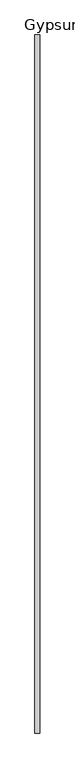
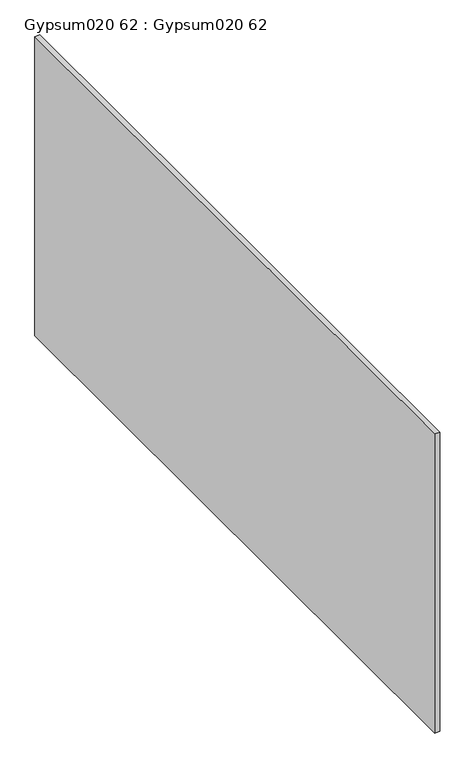
"""IFC4 building model written with IfcOpenShell, lengths in millimetres: proxy geometry, Gypsum020 62 : Gypsum020 62."""

import ifcopenshell
import ifcopenshell.guid

model = None  # the IFC model being written
_history = None  # IfcOwnerHistory: only IFC2X3 demands one
_inside = {}  # id of a spatial element -> (the spatial element, [elements in it])
_under = {}  # id of a project, library or spatial element -> (it, [spatial elements below it])
_declared = {}  # id of a project -> (the project, [libraries it declares])
_typed = {}  # id of a type object -> (the type object, [elements of that type])
_made_of = {}  # id of a material, layer set ... -> (it, [elements and type objects made of it])


def new_model(schema):
    """Start an empty IFC model of exactly this schema.

    Asked for "IFC4X3", IfcOpenShell would pick the latest addendum, in which some entities
    have other attributes; the version numbers below select the first issue.
    IFC2X3 requires an IfcOwnerHistory on every rooted entity: one is made here for all.
    """
    global model, _history
    if schema == "IFC4X3":
        model = ifcopenshell.file(schema_version=(4, 3, 0, 0))
    else:
        model = ifcopenshell.file(schema=schema)
    _inside.clear()
    _under.clear()
    _declared.clear()
    _typed.clear()
    _made_of.clear()
    _history = None
    if model.schema == "IFC2X3":
        org = make("IfcOrganization", Name="unknown")
        user = make(
            "IfcPersonAndOrganization",
            ThePerson=make("IfcPerson", FamilyName="unknown"),
            TheOrganization=org,
        )
        app = make(
            "IfcApplication",
            ApplicationDeveloper=org,
            Version="unknown",
            ApplicationFullName="unknown",
            ApplicationIdentifier="unknown",
        )
        _history = make(
            "IfcOwnerHistory",
            OwningUser=user,
            OwningApplication=app,
            ChangeAction="ADDED",
            CreationDate=0,
        )
    return model


def make(cls, **values):
    """One entity of the class cls with the attributes given. An attribute that is None is left unset."""
    return model.create_entity(
        cls, **{name: value for name, value in values.items() if value is not None}
    )


def rooted(cls, **values):
    """An entity with a GlobalId (a new one), such as an element, a storey or a relation."""
    return make(cls, GlobalId=ifcopenshell.guid.new(), OwnerHistory=_history, **values)


def si_unit(unit_type, name, prefix=None):
    """IfcSIUnit, for example si_unit("LENGTHUNIT", "METRE", prefix="MILLI")."""
    return make("IfcSIUnit", UnitType=unit_type, Prefix=prefix, Name=name)


def assignment(units):
    """IfcUnitAssignment: the units of a project."""
    return None if units is None else make("IfcUnitAssignment", Units=units)


def point(xyz):
    """IfcCartesianPoint."""
    return None if xyz is None else make("IfcCartesianPoint", Coordinates=xyz)


def direction(xyz):
    """IfcDirection."""
    return None if xyz is None else make("IfcDirection", DirectionRatios=xyz)


def frame(location, z_axis=None, x_axis=None):
    """IfcAxis2Placement3D, a coordinate frame: its origin and axes. An axis left out is left unset."""
    return make(
        "IfcAxis2Placement3D",
        Location=point(location),
        Axis=direction(z_axis),
        RefDirection=direction(x_axis),
    )


def origin():
    """The frame at (0, 0, 0) with its axes left unset."""
    return frame((0.0, 0.0, 0.0))


def place(relative_to, where):
    """IfcLocalPlacement: puts the frame where relative to a parent placement (None: the world)."""
    return make(
        "IfcLocalPlacement", PlacementRelTo=relative_to, RelativePlacement=where
    )


def context(
    kind, dimensions, precision=None, world=None, true_north=None, identifier=None
):
    """IfcGeometricRepresentationContext, for example the 3D "Model" context."""
    return make(
        "IfcGeometricRepresentationContext",
        ContextIdentifier=identifier,
        ContextType=kind,
        CoordinateSpaceDimension=dimensions,
        Precision=precision,
        WorldCoordinateSystem=world,
        TrueNorth=true_north,
    )


def project(units=None, contexts=None):
    """IfcProject with its units and contexts."""
    return rooted(
        "IfcProject",
        Name="project",
        RepresentationContexts=contexts,
        UnitsInContext=assignment(units),
    )


def spatial(cls, under=None, at=None, **own):
    """A site, building, storey or space (cls), placed at a placement, below another one or the project."""
    s = rooted(cls, ObjectPlacement=at, **own)
    if under is not None:
        _under.setdefault(under.id(), (under, []))[1].append(s)
    return s


def polyline(points):
    """IfcPolyline through the points."""
    return make("IfcPolyline", Points=[point(p) for p in points])


def outline(outer, holes=None, kind="AREA"):
    """IfcArbitraryClosedProfileDef: a profile drawn as a closed curve; with holes, ...WithVoids."""
    if holes is None:
        return make("IfcArbitraryClosedProfileDef", ProfileType=kind, OuterCurve=outer)
    return make(
        "IfcArbitraryProfileDefWithVoids",
        ProfileType=kind,
        OuterCurve=outer,
        InnerCurves=holes,
    )


def extrude(swept, where, along, depth):
    """IfcExtrudedAreaSolid: the profile swept, set in the frame where, extruded along a direction by depth."""
    return make(
        "IfcExtrudedAreaSolid",
        SweptArea=swept,
        Position=where,
        ExtrudedDirection=direction(along),
        Depth=depth,
    )


def shape(context_of_items, identifier, shape_type, items):
    """IfcShapeRepresentation: the items that make up one representation, for example the "Body"."""
    return make(
        "IfcShapeRepresentation",
        ContextOfItems=context_of_items,
        RepresentationIdentifier=identifier,
        RepresentationType=shape_type,
        Items=items,
    )


def source(mapping_origin, context_of_items, identifier, shape_type, items):
    """IfcRepresentationMap: a shape defined once, which mapped items show again and again."""
    return make(
        "IfcRepresentationMap",
        MappingOrigin=mapping_origin,
        MappedRepresentation=shape(context_of_items, identifier, shape_type, items),
    )


def transform(
    local_origin,
    x_axis=None,
    y_axis=None,
    z_axis=None,
    scale=None,
    scale2=None,
    scale3=None,
    uniform=True,
):
    """IfcCartesianTransformationOperator3D, or its non-uniform kind. x_axis, y_axis, z_axis: its Axis1, 2, 3."""
    if uniform:
        return make(
            "IfcCartesianTransformationOperator3D",
            Axis1=direction(x_axis),
            Axis2=direction(y_axis),
            LocalOrigin=point(local_origin),
            Scale=scale,
            Axis3=direction(z_axis),
        )
    return make(
        "IfcCartesianTransformationOperator3DnonUniform",
        Axis1=direction(x_axis),
        Axis2=direction(y_axis),
        LocalOrigin=point(local_origin),
        Scale=scale,
        Axis3=direction(z_axis),
        Scale2=scale2,
        Scale3=scale3,
    )


def mapped(mapping_source, mapping_target):
    """IfcMappedItem: shows the shape of a source again, moved by a transform."""
    return make(
        "IfcMappedItem", MappingSource=mapping_source, MappingTarget=mapping_target
    )


def made_of(thing, what):
    """Note that an element or type object is made of a material, layer set ...; save() writes the relation."""
    if what is not None:
        _made_of.setdefault(what.id(), (what, []))[1].append(thing)
    return thing


def element(
    cls,
    number,
    at=None,
    inside=None,
    cuts=None,
    type_object=None,
    material=None,
    context=None,
    identifier="Body",
    shape_type=None,
    held_by="IfcProductDefinitionShape",
    body=None,
    shapes=None,
    **own,
):
    """One element of the class cls, such as IfcWall. Its Tag is "e" and its number.

    at: its placement. inside: the storey or other place that contains it. cuts: it is an
    opening in that element (IfcRelVoidsElement). A single representation is given by context,
    identifier, shape_type and body (its items); several are given by shapes. held_by: the class
    of the entity that holds the representations. save() writes the other relations.
    """
    e = rooted(cls, Tag="e%d" % number, ObjectPlacement=at, **own)
    if body is not None:
        shapes = [shape(context, identifier, shape_type, body)]
    if shapes is not None:
        e.Representation = make(held_by, Representations=shapes)
    if inside is not None:
        _inside.setdefault(inside.id(), (inside, []))[1].append(e)
    if cuts is not None:
        rooted(
            "IfcRelVoidsElement", RelatingBuildingElement=cuts, RelatedOpeningElement=e
        )
    if type_object is not None:
        _typed.setdefault(type_object.id(), (type_object, []))[1].append(e)
    return made_of(e, material)


def aggregate(whole, parts):
    """IfcRelAggregates: a whole, such as a stair, and the parts it consists of."""
    return rooted("IfcRelAggregates", RelatingObject=whole, RelatedObjects=parts)


def save(model, path):
    """Write the relations noted so far, then the file.

    IfcRelAggregates (storeys below a building ...), IfcRelContainedInSpatialStructure (elements
    in a storey), IfcRelDefinesByType, IfcRelAssociatesMaterial and IfcRelDeclares: one each for
    every whole, place, type object, material and project.
    """
    for whole, parts in _under.values():
        aggregate(whole, parts)
    for where, things in _inside.values():
        rooted(
            "IfcRelContainedInSpatialStructure",
            RelatedElements=things,
            RelatingStructure=where,
        )
    for kind, things in _typed.values():
        rooted("IfcRelDefinesByType", RelatedObjects=things, RelatingType=kind)
    for what, things in _made_of.values():
        rooted("IfcRelAssociatesMaterial", RelatedObjects=things, RelatingMaterial=what)
    for by, libraries in _declared.values():
        rooted("IfcRelDeclares", RelatingContext=by, RelatedDefinitions=libraries)
    model.write(path)


def gypsum020_62_gypsum020_62_0a4c5181(model_context):
    return source(origin(), model_context, "Body", "SweptSolid", [
        extrude(outline(polyline([(-9487.2862014, 7982.1529269), (-9501.5737014, 7982.1529269), (-9501.5737014, 9982.1529269), (-9487.2862014, 9982.1529269), (-9487.2862014, 7982.1529269)])), frame((0.0, 0.0, 32619.6960253), z_axis=(0.0, 0.0, 1.0), x_axis=(1.0, 0.0, 0.0)), (0.0, 0.0, 1.0), 914.4000186),
    ])


if __name__ == "__main__":
    model = new_model("IFC4")
    model_context = context("Model", 3, world=origin())
    ifc_project = project(units=[si_unit("LENGTHUNIT", "METRE", prefix="MILLI")], contexts=[model_context])
    site = spatial("IfcSite", under=ifc_project)
    building = spatial("IfcBuilding", under=site)
    placement = place(None, origin())
    gypsum020_62_gypsum020_62_shape = gypsum020_62_gypsum020_62_0a4c5181(model_context)
    element("IfcBuildingElementProxy", 1, Name="Gypsum020 62 : Gypsum020 62", ObjectType="Gypsum020 62 : Gypsum020 62", at=placement, inside=building, context=model_context, shape_type="MappedRepresentation", body=[
        mapped(gypsum020_62_gypsum020_62_shape, transform((0.0, 0.0, 0.0), x_axis=(1.0, 0.0, 0.0), y_axis=(0.0, 1.0, 0.0), z_axis=(0.0, 0.0, 1.0))),
    ])
    save(model, "model.ifc")

# Revit data of these elements
# Type "Gypsum020 62 : Gypsum020 62"
#   NameOverride = "Gypsum020"
# Element 1 (IfcBuildingElementProxy, "Gypsum020 62 : Gypsum020 62")
#   Materials on its faces: "5/8\" GYPSUM BOARD"
# Materials
#   "5/8\" GYPSUM BOARD": class "Unassigned", colour RGB 255 255 255, transparency 0, Cost = 0
